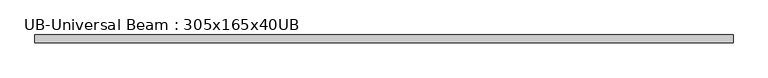
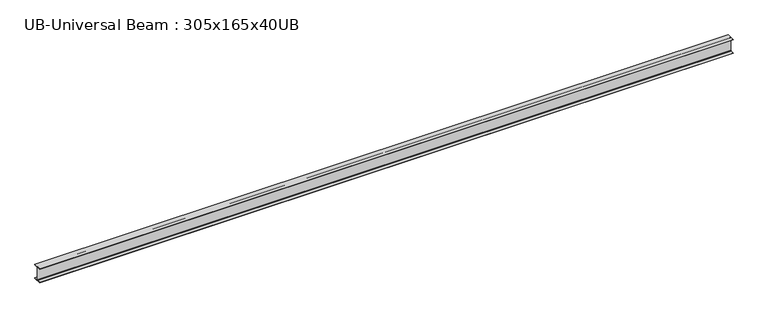
"""IFC4 building model written with IfcOpenShell, lengths in millimetres: beam geometry, UB-Universal Beam : 305x165x40UB."""

import ifcopenshell
import ifcopenshell.guid

model = None  # the IFC model being written
_history = None  # IfcOwnerHistory: only IFC2X3 demands one
_inside = {}  # id of a spatial element -> (the spatial element, [elements in it])
_under = {}  # id of a project, library or spatial element -> (it, [spatial elements below it])
_declared = {}  # id of a project -> (the project, [libraries it declares])
_typed = {}  # id of a type object -> (the type object, [elements of that type])
_made_of = {}  # id of a material, layer set ... -> (it, [elements and type objects made of it])


def new_model(schema):
    """Start an empty IFC model of exactly this schema.

    Asked for "IFC4X3", IfcOpenShell would pick the latest addendum, in which some entities
    have other attributes; the version numbers below select the first issue.
    IFC2X3 requires an IfcOwnerHistory on every rooted entity: one is made here for all.
    """
    global model, _history
    if schema == "IFC4X3":
        model = ifcopenshell.file(schema_version=(4, 3, 0, 0))
    else:
        model = ifcopenshell.file(schema=schema)
    _inside.clear()
    _under.clear()
    _declared.clear()
    _typed.clear()
    _made_of.clear()
    _history = None
    if model.schema == "IFC2X3":
        org = make("IfcOrganization", Name="unknown")
        user = make(
            "IfcPersonAndOrganization",
            ThePerson=make("IfcPerson", FamilyName="unknown"),
            TheOrganization=org,
        )
        app = make(
            "IfcApplication",
            ApplicationDeveloper=org,
            Version="unknown",
            ApplicationFullName="unknown",
            ApplicationIdentifier="unknown",
        )
        _history = make(
            "IfcOwnerHistory",
            OwningUser=user,
            OwningApplication=app,
            ChangeAction="ADDED",
            CreationDate=0,
        )
    return model


def make(cls, **values):
    """One entity of the class cls with the attributes given. An attribute that is None is left unset."""
    return model.create_entity(
        cls, **{name: value for name, value in values.items() if value is not None}
    )


def rooted(cls, **values):
    """An entity with a GlobalId (a new one), such as an element, a storey or a relation."""
    return make(cls, GlobalId=ifcopenshell.guid.new(), OwnerHistory=_history, **values)


def si_unit(unit_type, name, prefix=None):
    """IfcSIUnit, for example si_unit("LENGTHUNIT", "METRE", prefix="MILLI")."""
    return make("IfcSIUnit", UnitType=unit_type, Prefix=prefix, Name=name)


def assignment(units):
    """IfcUnitAssignment: the units of a project."""
    return None if units is None else make("IfcUnitAssignment", Units=units)


def point(xyz):
    """IfcCartesianPoint."""
    return None if xyz is None else make("IfcCartesianPoint", Coordinates=xyz)


def direction(xyz):
    """IfcDirection."""
    return None if xyz is None else make("IfcDirection", DirectionRatios=xyz)


def frame(location, z_axis=None, x_axis=None):
    """IfcAxis2Placement3D, a coordinate frame: its origin and axes. An axis left out is left unset."""
    return make(
        "IfcAxis2Placement3D",
        Location=point(location),
        Axis=direction(z_axis),
        RefDirection=direction(x_axis),
    )


def frame_2d(location, x_axis=None):
    """IfcAxis2Placement2D, a coordinate frame in the plane: its origin and x axis."""
    return make(
        "IfcAxis2Placement2D", Location=point(location), RefDirection=direction(x_axis)
    )


def origin():
    """The frame at (0, 0, 0) with its axes left unset."""
    return frame((0.0, 0.0, 0.0))


def place(relative_to, where):
    """IfcLocalPlacement: puts the frame where relative to a parent placement (None: the world)."""
    return make(
        "IfcLocalPlacement", PlacementRelTo=relative_to, RelativePlacement=where
    )


def context(
    kind, dimensions, precision=None, world=None, true_north=None, identifier=None
):
    """IfcGeometricRepresentationContext, for example the 3D "Model" context."""
    return make(
        "IfcGeometricRepresentationContext",
        ContextIdentifier=identifier,
        ContextType=kind,
        CoordinateSpaceDimension=dimensions,
        Precision=precision,
        WorldCoordinateSystem=world,
        TrueNorth=true_north,
    )


def project(units=None, contexts=None):
    """IfcProject with its units and contexts."""
    return rooted(
        "IfcProject",
        Name="project",
        RepresentationContexts=contexts,
        UnitsInContext=assignment(units),
    )


def spatial(cls, under=None, at=None, **own):
    """A site, building, storey or space (cls), placed at a placement, below another one or the project."""
    s = rooted(cls, ObjectPlacement=at, **own)
    if under is not None:
        _under.setdefault(under.id(), (under, []))[1].append(s)
    return s


def polyline(points):
    """IfcPolyline through the points."""
    return make("IfcPolyline", Points=[point(p) for p in points])


def circle_curve(where, radius):
    """IfcCircle in the frame where."""
    return make("IfcCircle", Position=where, Radius=radius)


def trimmed(basis, trim1, trim2, sense, master):
    """IfcTrimmedCurve: the piece of a basis curve between two trims."""
    return make(
        "IfcTrimmedCurve",
        BasisCurve=basis,
        Trim1=trim1,
        Trim2=trim2,
        SenseAgreement=sense,
        MasterRepresentation=master,
    )


def segment(curve, same_sense, transition):
    """IfcCompositeCurveSegment."""
    return make(
        "IfcCompositeCurveSegment",
        Transition=transition,
        SameSense=same_sense,
        ParentCurve=curve,
    )


def composite_curve(segments, self_intersect=None):
    """IfcCompositeCurve: segments joined end to end."""
    return make("IfcCompositeCurve", Segments=segments, SelfIntersect=self_intersect)


def outline(outer, holes=None, kind="AREA"):
    """IfcArbitraryClosedProfileDef: a profile drawn as a closed curve; with holes, ...WithVoids."""
    if holes is None:
        return make("IfcArbitraryClosedProfileDef", ProfileType=kind, OuterCurve=outer)
    return make(
        "IfcArbitraryProfileDefWithVoids",
        ProfileType=kind,
        OuterCurve=outer,
        InnerCurves=holes,
    )


def extrude(swept, where, along, depth):
    """IfcExtrudedAreaSolid: the profile swept, set in the frame where, extruded along a direction by depth."""
    return make(
        "IfcExtrudedAreaSolid",
        SweptArea=swept,
        Position=where,
        ExtrudedDirection=direction(along),
        Depth=depth,
    )


def shape(context_of_items, identifier, shape_type, items):
    """IfcShapeRepresentation: the items that make up one representation, for example the "Body"."""
    return make(
        "IfcShapeRepresentation",
        ContextOfItems=context_of_items,
        RepresentationIdentifier=identifier,
        RepresentationType=shape_type,
        Items=items,
    )


def source(mapping_origin, context_of_items, identifier, shape_type, items):
    """IfcRepresentationMap: a shape defined once, which mapped items show again and again."""
    return make(
        "IfcRepresentationMap",
        MappingOrigin=mapping_origin,
        MappedRepresentation=shape(context_of_items, identifier, shape_type, items),
    )


def transform(
    local_origin,
    x_axis=None,
    y_axis=None,
    z_axis=None,
    scale=None,
    scale2=None,
    scale3=None,
    uniform=True,
):
    """IfcCartesianTransformationOperator3D, or its non-uniform kind. x_axis, y_axis, z_axis: its Axis1, 2, 3."""
    if uniform:
        return make(
            "IfcCartesianTransformationOperator3D",
            Axis1=direction(x_axis),
            Axis2=direction(y_axis),
            LocalOrigin=point(local_origin),
            Scale=scale,
            Axis3=direction(z_axis),
        )
    return make(
        "IfcCartesianTransformationOperator3DnonUniform",
        Axis1=direction(x_axis),
        Axis2=direction(y_axis),
        LocalOrigin=point(local_origin),
        Scale=scale,
        Axis3=direction(z_axis),
        Scale2=scale2,
        Scale3=scale3,
    )


def mapped(mapping_source, mapping_target):
    """IfcMappedItem: shows the shape of a source again, moved by a transform."""
    return make(
        "IfcMappedItem", MappingSource=mapping_source, MappingTarget=mapping_target
    )


def made_of(thing, what):
    """Note that an element or type object is made of a material, layer set ...; save() writes the relation."""
    if what is not None:
        _made_of.setdefault(what.id(), (what, []))[1].append(thing)
    return thing


def element(
    cls,
    number,
    at=None,
    inside=None,
    cuts=None,
    type_object=None,
    material=None,
    context=None,
    identifier="Body",
    shape_type=None,
    held_by="IfcProductDefinitionShape",
    body=None,
    shapes=None,
    **own,
):
    """One element of the class cls, such as IfcWall. Its Tag is "e" and its number.

    at: its placement. inside: the storey or other place that contains it. cuts: it is an
    opening in that element (IfcRelVoidsElement). A single representation is given by context,
    identifier, shape_type and body (its items); several are given by shapes. held_by: the class
    of the entity that holds the representations. save() writes the other relations.
    """
    e = rooted(cls, Tag="e%d" % number, ObjectPlacement=at, **own)
    if body is not None:
        shapes = [shape(context, identifier, shape_type, body)]
    if shapes is not None:
        e.Representation = make(held_by, Representations=shapes)
    if inside is not None:
        _inside.setdefault(inside.id(), (inside, []))[1].append(e)
    if cuts is not None:
        rooted(
            "IfcRelVoidsElement", RelatingBuildingElement=cuts, RelatedOpeningElement=e
        )
    if type_object is not None:
        _typed.setdefault(type_object.id(), (type_object, []))[1].append(e)
    return made_of(e, material)


def aggregate(whole, parts):
    """IfcRelAggregates: a whole, such as a stair, and the parts it consists of."""
    return rooted("IfcRelAggregates", RelatingObject=whole, RelatedObjects=parts)


def save(model, path):
    """Write the relations noted so far, then the file.

    IfcRelAggregates (storeys below a building ...), IfcRelContainedInSpatialStructure (elements
    in a storey), IfcRelDefinesByType, IfcRelAssociatesMaterial and IfcRelDeclares: one each for
    every whole, place, type object, material and project.
    """
    for whole, parts in _under.values():
        aggregate(whole, parts)
    for where, things in _inside.values():
        rooted(
            "IfcRelContainedInSpatialStructure",
            RelatedElements=things,
            RelatingStructure=where,
        )
    for kind, things in _typed.values():
        rooted("IfcRelDefinesByType", RelatedObjects=things, RelatingType=kind)
    for what, things in _made_of.values():
        rooted("IfcRelAssociatesMaterial", RelatedObjects=things, RelatingMaterial=what)
    for by, libraries in _declared.values():
        rooted("IfcRelDeclares", RelatingContext=by, RelatedDefinitions=libraries)
    model.write(path)


def ub_universal_beam_305x165x40ub_f67fc52f(model_context):
    return source(origin(), model_context, "Body", "SweptSolid", [
        extrude(outline(composite_curve([segment(polyline([(82.5, -141.5), (82.5, -151.7), (-82.5, -151.7), (-82.5, -141.5), (-11.9, -141.5)]), True, "CONTINUOUS"), segment(trimmed(circle_curve(frame_2d((-11.9, -132.6)), 8.9), [point((-11.9, -141.5))], [point((-3.0, -132.6))], True, "CARTESIAN"), True, "CONTINUOUS"), segment(polyline([(-3.0, -132.6), (-3.0, 132.6)]), True, "CONTINUOUS"), segment(trimmed(circle_curve(frame_2d((-11.9, 132.6)), 8.9), [point((-3.0, 132.6))], [point((-11.9, 141.5))], True, "CARTESIAN"), True, "CONTINUOUS"), segment(polyline([(-11.9, 141.5), (-82.5, 141.5), (-82.5, 151.7), (82.5, 151.7), (82.5, 141.5), (11.9, 141.5)]), True, "CONTINUOUS"), segment(trimmed(circle_curve(frame_2d((11.9, 132.6)), 8.9), [point((11.9, 141.5))], [point((3.0, 132.6))], True, "CARTESIAN"), True, "CONTINUOUS"), segment(polyline([(3.0, 132.6), (3.0, -132.6)]), True, "CONTINUOUS"), segment(trimmed(circle_curve(frame_2d((11.9, -132.6)), 8.9), [point((3.0, -132.6))], [point((11.9, -141.5))], True, "CARTESIAN"), True, "CONTINUOUS"), segment(polyline([(11.9, -141.5), (82.5, -141.5)]), True, "CONTINUOUS")], self_intersect=False)), frame((-7125.0, 0.0, 0.0), z_axis=(1.0, 0.0, 0.0), x_axis=(0.0, 1.0, 0.0)), (0.0, 0.0, 1.0), 14250.0),
    ])


if __name__ == "__main__":
    model = new_model("IFC4")
    model_context = context("Model", 3, world=origin())
    ifc_project = project(units=[si_unit("LENGTHUNIT", "METRE", prefix="MILLI")], contexts=[model_context])
    site = spatial("IfcSite", under=ifc_project)
    building = spatial("IfcBuilding", under=site)
    placement = place(None, origin())
    ub_universal_beam_305x165x40ub_shape = ub_universal_beam_305x165x40ub_f67fc52f(model_context)
    element("IfcBeam", 1, ObjectType="UB-Universal Beam : 305x165x40UB", at=placement, inside=building, context=model_context, shape_type="MappedRepresentation", body=[
        mapped(ub_universal_beam_305x165x40ub_shape, transform((0.0, 0.0, 0.0), x_axis=(1.0, 0.0, 0.0), y_axis=(0.0, 1.0, 0.0), z_axis=(0.0, 0.0, 1.0))),
    ])
    save(model, "model.ifc")

# Revit data of these elements
# Type "UB-Universal Beam : 305x165x40UB"
#   Nominal h = "305"
#   W = 0
#   Start Extension Calculation [instance default] = 3000 mm
#   Start Extension [instance default] = -12.7 mm
#   End Extension Calculation [instance default] = 3000 mm
#   End Extension [instance default] = -12.7 mm
#   Ix = 8503
#   Length [instance default] = 1524 mm
#   M = 40.3
#   Zx = 560
#   b = 165 mm
#   h = 303.4 mm
#   r = 8.9 mm
#   s = 6 mm
#   t = 10.2 mm
#   A = 0.005 m²
#   Structural Material [instance default] = Metal - Steel - 345 MPa
#   Assembly Code = ""
# Element 1 (IfcBeam, "UB-Universal Beam : 305x165x40UB")
#   Materials on its faces: "Metal - Steel - 345 MPa"
# Materials
#   "Metal - Steel - 345 MPa": class "Metal", colour RGB 241 46 46, transparency 0
